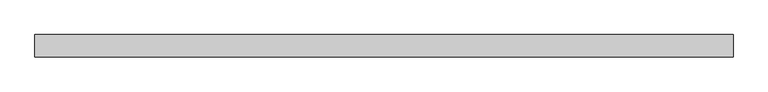
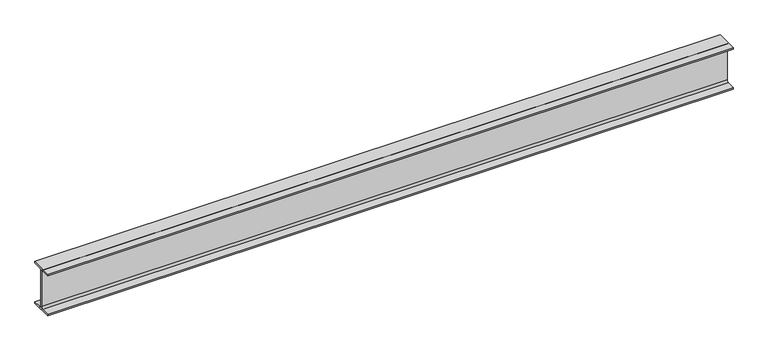
"""IFC4 building model written with IfcOpenShell, lengths in millimetres: beam geometry, 0912_Steel Framing_H-KSD3502 : H_SB_ASB_H-250x125x6x9."""

import ifcopenshell
import ifcopenshell.guid

model = None  # the IFC model being written
_history = None  # IfcOwnerHistory: only IFC2X3 demands one
_inside = {}  # id of a spatial element -> (the spatial element, [elements in it])
_under = {}  # id of a project, library or spatial element -> (it, [spatial elements below it])
_declared = {}  # id of a project -> (the project, [libraries it declares])
_typed = {}  # id of a type object -> (the type object, [elements of that type])
_made_of = {}  # id of a material, layer set ... -> (it, [elements and type objects made of it])


def new_model(schema):
    """Start an empty IFC model of exactly this schema.

    Asked for "IFC4X3", IfcOpenShell would pick the latest addendum, in which some entities
    have other attributes; the version numbers below select the first issue.
    IFC2X3 requires an IfcOwnerHistory on every rooted entity: one is made here for all.
    """
    global model, _history
    if schema == "IFC4X3":
        model = ifcopenshell.file(schema_version=(4, 3, 0, 0))
    else:
        model = ifcopenshell.file(schema=schema)
    _inside.clear()
    _under.clear()
    _declared.clear()
    _typed.clear()
    _made_of.clear()
    _history = None
    if model.schema == "IFC2X3":
        org = make("IfcOrganization", Name="unknown")
        user = make(
            "IfcPersonAndOrganization",
            ThePerson=make("IfcPerson", FamilyName="unknown"),
            TheOrganization=org,
        )
        app = make(
            "IfcApplication",
            ApplicationDeveloper=org,
            Version="unknown",
            ApplicationFullName="unknown",
            ApplicationIdentifier="unknown",
        )
        _history = make(
            "IfcOwnerHistory",
            OwningUser=user,
            OwningApplication=app,
            ChangeAction="ADDED",
            CreationDate=0,
        )
    return model


def make(cls, **values):
    """One entity of the class cls with the attributes given. An attribute that is None is left unset."""
    return model.create_entity(
        cls, **{name: value for name, value in values.items() if value is not None}
    )


def rooted(cls, **values):
    """An entity with a GlobalId (a new one), such as an element, a storey or a relation."""
    return make(cls, GlobalId=ifcopenshell.guid.new(), OwnerHistory=_history, **values)


def si_unit(unit_type, name, prefix=None):
    """IfcSIUnit, for example si_unit("LENGTHUNIT", "METRE", prefix="MILLI")."""
    return make("IfcSIUnit", UnitType=unit_type, Prefix=prefix, Name=name)


def assignment(units):
    """IfcUnitAssignment: the units of a project."""
    return None if units is None else make("IfcUnitAssignment", Units=units)


def point(xyz):
    """IfcCartesianPoint."""
    return None if xyz is None else make("IfcCartesianPoint", Coordinates=xyz)


def direction(xyz):
    """IfcDirection."""
    return None if xyz is None else make("IfcDirection", DirectionRatios=xyz)


def frame(location, z_axis=None, x_axis=None):
    """IfcAxis2Placement3D, a coordinate frame: its origin and axes. An axis left out is left unset."""
    return make(
        "IfcAxis2Placement3D",
        Location=point(location),
        Axis=direction(z_axis),
        RefDirection=direction(x_axis),
    )


def frame_2d(location, x_axis=None):
    """IfcAxis2Placement2D, a coordinate frame in the plane: its origin and x axis."""
    return make(
        "IfcAxis2Placement2D", Location=point(location), RefDirection=direction(x_axis)
    )


def origin():
    """The frame at (0, 0, 0) with its axes left unset."""
    return frame((0.0, 0.0, 0.0))


def place(relative_to, where):
    """IfcLocalPlacement: puts the frame where relative to a parent placement (None: the world)."""
    return make(
        "IfcLocalPlacement", PlacementRelTo=relative_to, RelativePlacement=where
    )


def context(
    kind, dimensions, precision=None, world=None, true_north=None, identifier=None
):
    """IfcGeometricRepresentationContext, for example the 3D "Model" context."""
    return make(
        "IfcGeometricRepresentationContext",
        ContextIdentifier=identifier,
        ContextType=kind,
        CoordinateSpaceDimension=dimensions,
        Precision=precision,
        WorldCoordinateSystem=world,
        TrueNorth=true_north,
    )


def project(units=None, contexts=None):
    """IfcProject with its units and contexts."""
    return rooted(
        "IfcProject",
        Name="project",
        RepresentationContexts=contexts,
        UnitsInContext=assignment(units),
    )


def spatial(cls, under=None, at=None, **own):
    """A site, building, storey or space (cls), placed at a placement, below another one or the project."""
    s = rooted(cls, ObjectPlacement=at, **own)
    if under is not None:
        _under.setdefault(under.id(), (under, []))[1].append(s)
    return s


def polyline(points):
    """IfcPolyline through the points."""
    return make("IfcPolyline", Points=[point(p) for p in points])


def circle_curve(where, radius):
    """IfcCircle in the frame where."""
    return make("IfcCircle", Position=where, Radius=radius)


def trimmed(basis, trim1, trim2, sense, master):
    """IfcTrimmedCurve: the piece of a basis curve between two trims."""
    return make(
        "IfcTrimmedCurve",
        BasisCurve=basis,
        Trim1=trim1,
        Trim2=trim2,
        SenseAgreement=sense,
        MasterRepresentation=master,
    )


def segment(curve, same_sense, transition):
    """IfcCompositeCurveSegment."""
    return make(
        "IfcCompositeCurveSegment",
        Transition=transition,
        SameSense=same_sense,
        ParentCurve=curve,
    )


def composite_curve(segments, self_intersect=None):
    """IfcCompositeCurve: segments joined end to end."""
    return make("IfcCompositeCurve", Segments=segments, SelfIntersect=self_intersect)


def outline(outer, holes=None, kind="AREA"):
    """IfcArbitraryClosedProfileDef: a profile drawn as a closed curve; with holes, ...WithVoids."""
    if holes is None:
        return make("IfcArbitraryClosedProfileDef", ProfileType=kind, OuterCurve=outer)
    return make(
        "IfcArbitraryProfileDefWithVoids",
        ProfileType=kind,
        OuterCurve=outer,
        InnerCurves=holes,
    )


def extrude(swept, where, along, depth):
    """IfcExtrudedAreaSolid: the profile swept, set in the frame where, extruded along a direction by depth."""
    return make(
        "IfcExtrudedAreaSolid",
        SweptArea=swept,
        Position=where,
        ExtrudedDirection=direction(along),
        Depth=depth,
    )


def shape(context_of_items, identifier, shape_type, items):
    """IfcShapeRepresentation: the items that make up one representation, for example the "Body"."""
    return make(
        "IfcShapeRepresentation",
        ContextOfItems=context_of_items,
        RepresentationIdentifier=identifier,
        RepresentationType=shape_type,
        Items=items,
    )


def source(mapping_origin, context_of_items, identifier, shape_type, items):
    """IfcRepresentationMap: a shape defined once, which mapped items show again and again."""
    return make(
        "IfcRepresentationMap",
        MappingOrigin=mapping_origin,
        MappedRepresentation=shape(context_of_items, identifier, shape_type, items),
    )


def transform(
    local_origin,
    x_axis=None,
    y_axis=None,
    z_axis=None,
    scale=None,
    scale2=None,
    scale3=None,
    uniform=True,
):
    """IfcCartesianTransformationOperator3D, or its non-uniform kind. x_axis, y_axis, z_axis: its Axis1, 2, 3."""
    if uniform:
        return make(
            "IfcCartesianTransformationOperator3D",
            Axis1=direction(x_axis),
            Axis2=direction(y_axis),
            LocalOrigin=point(local_origin),
            Scale=scale,
            Axis3=direction(z_axis),
        )
    return make(
        "IfcCartesianTransformationOperator3DnonUniform",
        Axis1=direction(x_axis),
        Axis2=direction(y_axis),
        LocalOrigin=point(local_origin),
        Scale=scale,
        Axis3=direction(z_axis),
        Scale2=scale2,
        Scale3=scale3,
    )


def mapped(mapping_source, mapping_target):
    """IfcMappedItem: shows the shape of a source again, moved by a transform."""
    return make(
        "IfcMappedItem", MappingSource=mapping_source, MappingTarget=mapping_target
    )


def made_of(thing, what):
    """Note that an element or type object is made of a material, layer set ...; save() writes the relation."""
    if what is not None:
        _made_of.setdefault(what.id(), (what, []))[1].append(thing)
    return thing


def element(
    cls,
    number,
    at=None,
    inside=None,
    cuts=None,
    type_object=None,
    material=None,
    context=None,
    identifier="Body",
    shape_type=None,
    held_by="IfcProductDefinitionShape",
    body=None,
    shapes=None,
    **own,
):
    """One element of the class cls, such as IfcWall. Its Tag is "e" and its number.

    at: its placement. inside: the storey or other place that contains it. cuts: it is an
    opening in that element (IfcRelVoidsElement). A single representation is given by context,
    identifier, shape_type and body (its items); several are given by shapes. held_by: the class
    of the entity that holds the representations. save() writes the other relations.
    """
    e = rooted(cls, Tag="e%d" % number, ObjectPlacement=at, **own)
    if body is not None:
        shapes = [shape(context, identifier, shape_type, body)]
    if shapes is not None:
        e.Representation = make(held_by, Representations=shapes)
    if inside is not None:
        _inside.setdefault(inside.id(), (inside, []))[1].append(e)
    if cuts is not None:
        rooted(
            "IfcRelVoidsElement", RelatingBuildingElement=cuts, RelatedOpeningElement=e
        )
    if type_object is not None:
        _typed.setdefault(type_object.id(), (type_object, []))[1].append(e)
    return made_of(e, material)


def aggregate(whole, parts):
    """IfcRelAggregates: a whole, such as a stair, and the parts it consists of."""
    return rooted("IfcRelAggregates", RelatingObject=whole, RelatedObjects=parts)


def save(model, path):
    """Write the relations noted so far, then the file.

    IfcRelAggregates (storeys below a building ...), IfcRelContainedInSpatialStructure (elements
    in a storey), IfcRelDefinesByType, IfcRelAssociatesMaterial and IfcRelDeclares: one each for
    every whole, place, type object, material and project.
    """
    for whole, parts in _under.values():
        aggregate(whole, parts)
    for where, things in _inside.values():
        rooted(
            "IfcRelContainedInSpatialStructure",
            RelatedElements=things,
            RelatingStructure=where,
        )
    for kind, things in _typed.values():
        rooted("IfcRelDefinesByType", RelatedObjects=things, RelatingType=kind)
    for what, things in _made_of.values():
        rooted("IfcRelAssociatesMaterial", RelatedObjects=things, RelatingMaterial=what)
    for by, libraries in _declared.values():
        rooted("IfcRelDeclares", RelatingContext=by, RelatedDefinitions=libraries)
    model.write(path)


def beam_1ee0d709(model_context):
    return source(origin(), model_context, "Body", "SweptSolid", [
        extrude(outline(composite_curve([segment(polyline([(62.5, -116.0), (62.5, -125.0), (-62.5, -125.0), (-62.5, -116.0), (-15.0, -116.0)]), True, "CONTINUOUS"), segment(trimmed(circle_curve(frame_2d((-15.0, -104.0)), 12.0), [point((-15.0, -116.0))], [point((-3.0, -104.0))], True, "CARTESIAN"), True, "CONTINUOUS"), segment(polyline([(-3.0, -104.0), (-3.0, 104.0)]), True, "CONTINUOUS"), segment(trimmed(circle_curve(frame_2d((-15.0, 104.0)), 12.0), [point((-3.0, 104.0))], [point((-15.0, 116.0))], True, "CARTESIAN"), True, "CONTINUOUS"), segment(polyline([(-15.0, 116.0), (-62.5, 116.0), (-62.5, 125.0), (62.5, 125.0), (62.5, 116.0), (15.0, 116.0)]), True, "CONTINUOUS"), segment(trimmed(circle_curve(frame_2d((15.0, 104.0)), 12.0), [point((15.0, 116.0))], [point((3.0, 104.0))], True, "CARTESIAN"), True, "CONTINUOUS"), segment(polyline([(3.0, 104.0), (3.0, -104.0)]), True, "CONTINUOUS"), segment(trimmed(circle_curve(frame_2d((15.0, -104.0)), 12.0), [point((3.0, -104.0))], [point((15.0, -116.0))], True, "CARTESIAN"), True, "CONTINUOUS"), segment(polyline([(15.0, -116.0), (62.5, -116.0)]), True, "CONTINUOUS")], self_intersect=False)), frame((-1904.8, 0.0, 0.0), z_axis=(1.0, 0.0, 0.0), x_axis=(0.0, 1.0, 0.0)), (0.0, 0.0, 1.0), 3892.0999994),
    ])


if __name__ == "__main__":
    model = new_model("IFC4")
    model_context = context("Model", 3, world=origin())
    ifc_project = project(units=[si_unit("LENGTHUNIT", "METRE", prefix="MILLI")], contexts=[model_context])
    site = spatial("IfcSite", under=ifc_project)
    building = spatial("IfcBuilding", under=site)
    placement = place(None, origin())
    beam_shape = beam_1ee0d709(model_context)
    element("IfcBeam", 1, ObjectType="0912_Steel Framing_H-KSD3502 : H_SB_ASB_H-250x125x6x9", at=placement, inside=building, context=model_context, shape_type="MappedRepresentation", body=[
        mapped(beam_shape, transform((0.0, 0.0, 0.0), x_axis=(1.0, 0.0, 0.0), y_axis=(0.0, 1.0, 0.0), z_axis=(0.0, 0.0, 1.0))),
    ])
    save(model, "model.ifc")

# Revit data of these elements
# Type "0912_Steel Framing_H-KSD3502 : H_SB_ASB_H-250x125x6x9"
#   H_WM Code_1 = "S01AA003-00001 | Main Steel Structure Fabrication Work | Shelter/Building | Light Steel - Standard (30KG/M>Weight) | Material: (   )"
#   H_WM Code_2 = "S03AA029-00001 | Main Steel Structure Erection Work | Shelter/Building | Light Steel (30KG/M>Weight) | Material: (   )"
#   H_WM Code_3 = "S01AA010-00001 | Main Steel Structure Fabrication Work | Shelter/Building | Steel Painting/Coating | for Non-Fireproofed Steel Surface, Surface Preparation, Primer, Second & Final Coat | Material: (   )"
#   H_Q'ty Cal Type Tag = "SB-Q2"
#   Width = 12.5 cm
#   Web Thickness = 0.6 cm
#   Web Fillet = 1.2 cm
#   Warping Constant = 42539.8 cm⁶
#   W = 0
#   Torsional Moment of Inertia = 7.8102 cm⁴
#   Section Area = 37.66 cm²
#   Plastic Modulus weak axis = 73.1 cm³
#   Plastic Modulus strong axis = 366.0 cm³
#   Perimeter = 0.97 m²/m
#   Nominal Weight = 29.60 kgf/m
#   Moment of Inertia weak axis = 294.00 cm⁴
#   Moment of Inertia strong axis = 4050.00 cm⁴
#   Height = 25.0 cm
#   Flange Thickness = 0.9 cm
#   Elastic Modulus weak axis = 47.0 cm³
#   Elastic Modulus strong axis = 324.0 cm³
#   Centroid Vertical = 12.5 cm
#   Centroid Horizontal = 6.25 cm
#   Ix = 40500000
#   Length [instance default] = 1.5240 m
#   Zx = 366000
#   b = 0.1250 m
#   h = 0.2500 m
#   r = 0.0120 m
#   s = 0.0060 m
#   t = 0.0090 m
#   A = 0.003766 m²
#   Structural Material [instance default] = Steel, 45-345
#   Assembly Code = ""
# Element 1 (IfcBeam, "0912_Steel Framing_H-KSD3502 : H_SB_ASB_H-250x125x6x9")
#   Structural Material = none
# Materials
#   "Steel, 45-345": class "Metal", colour RGB 189 187 185, transparency 0, Description = "Steel 345 MPa", Cost = 0
